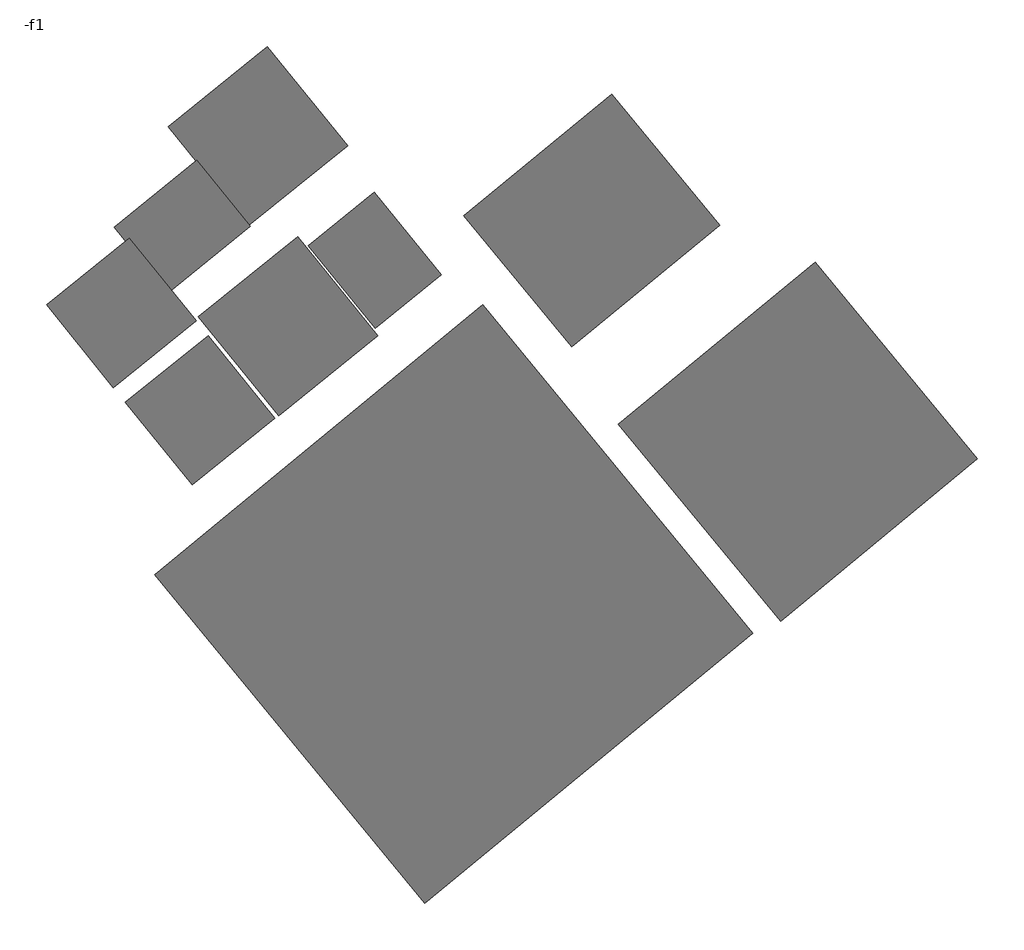
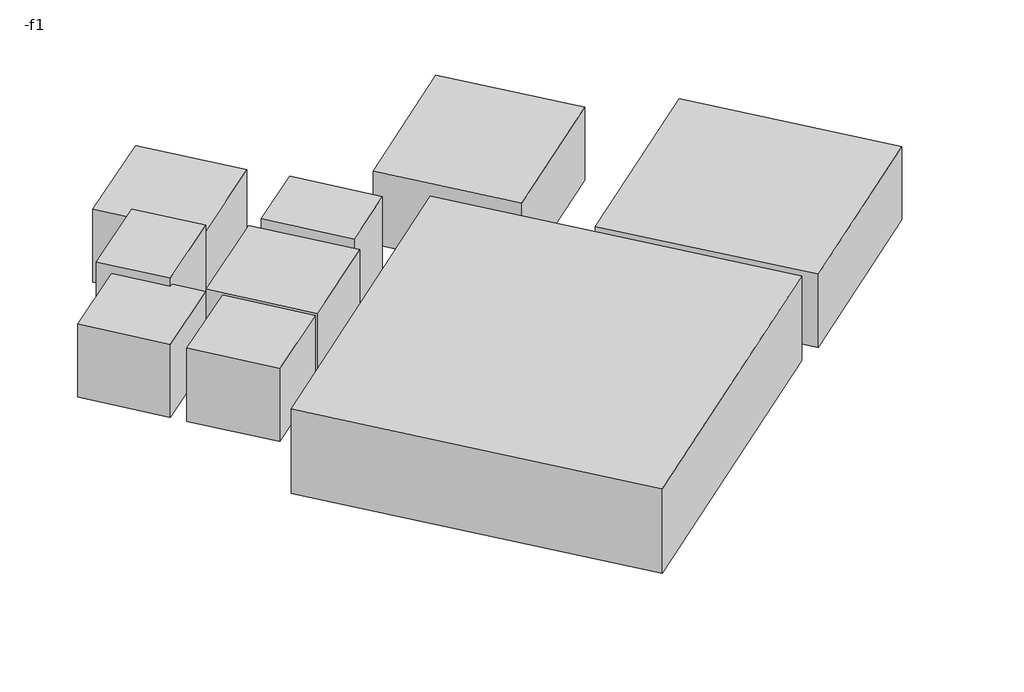
# One storey: 9 proxies.
"""IFC4 building model written with IfcOpenShell, lengths in millimetres."""

from ifc_helpers import new_model, si_unit, frame, origin, place, context, project, spatial, polyline, outline, extrude, element, save

model = new_model("IFC4")

# Units and contexts
model_context = context("Model", 3, world=origin())
ifc_project = project(units=[si_unit("LENGTHUNIT", "METRE", prefix="MILLI")], contexts=[model_context])

# Site, building, storey
site = spatial("IfcSite", under=ifc_project)
building = spatial("IfcBuilding", under=site)
storey = spatial("IfcBuildingStorey", under=building, Name="-f1", Elevation=-1400.0)

# Proxies
placement = place(None, origin())
element("IfcBuildingElementProxy", 1, Name="私有-封闭 : Supply, Equipment, and Seasonal Furniture Storage", ObjectType="私有-封闭 : Supply, Equipment, and Seasonal Furniture Storage", at=placement, inside=storey, context=model_context, shape_type="SweptSolid", body=[
    extrude(outline(polyline([(-34794.6694804, 4511.352913), (-31018.7471341, -151.5228557), (-35681.6229029, -3927.445202), (-39457.5452492, 735.4305667), (-34794.6694804, 4511.352913)])), frame((0.0, 0.0, -1400.0), z_axis=(0.0, 0.0, 1.0), x_axis=(1.0, 0.0, 0.0)), (0.0, 0.0, 1.0), 4500.0),
])
element("IfcBuildingElementProxy", 2, Name="私有-封闭 : Landscape and Grounds Maintenance Equipment Storage", ObjectType="私有-封闭 : Landscape and Grounds Maintenance Equipment Storage", at=placement, inside=storey, context=model_context, shape_type="SweptSolid", body=[
    extrude(outline(polyline([(-39005.8178352, -144.9924785), (-35859.2158799, -4030.7222858), (-39744.9456872, -7177.3242411), (-42891.5476425, -3291.5944338), (-39005.8178352, -144.9924785)])), frame((0.0, 0.0, -1400.0), z_axis=(0.0, 0.0, 1.0), x_axis=(1.0, 0.0, 0.0)), (0.0, 0.0, 1.0), 4500.0),
])
element("IfcBuildingElementProxy", 3, Name="临时私有-开敞 : IT Server, Workroom and Staff Offices", ObjectType="临时私有-开敞 : IT Server, Workroom and Staff Offices", at=placement, inside=storey, context=model_context, shape_type="SweptSolid", body=[
    extrude(outline(polyline([(-36216.5856453, 13452.3157929), (-32440.663299, 8789.4400242), (-37103.5390677, 5013.5176779), (-40879.461414, 9676.3934466), (-36216.5856453, 13452.3157929)])), frame((0.0, 0.0, -1400.0), z_axis=(0.0, 0.0, 1.0), x_axis=(1.0, 0.0, 0.0)), (0.0, 0.0, 1.0), 4500.0),
])
element("IfcBuildingElementProxy", 4, Name="临时私有-开敞 : Custodial Office", ObjectType="临时私有-开敞 : Custodial Office", at=placement, inside=storey, context=model_context, shape_type="SweptSolid", body=[
    extrude(outline(polyline([(-39531.1745049, 8096.0214901), (-37013.8929407, 4987.4376443), (-40899.622748, 1840.835689), (-43416.9043122, 4949.4195349), (-39531.1745049, 8096.0214901)])), frame((0.0, 0.0, -1400.0), z_axis=(0.0, 0.0, 1.0), x_axis=(1.0, 0.0, 0.0)), (0.0, 0.0, 1.0), 5000.0),
])
element("IfcBuildingElementProxy", 5, Name="私有-封闭 : Electrical", ObjectType="私有-封闭 : Electrical", at=placement, inside=storey, context=model_context, shape_type="SweptSolid", body=[
    extrude(outline(polyline([(-20018.4686757, 11213.5389154), (-14935.0026254, 5036.2925292), (-21884.4048099, -682.6067774), (-26967.8708601, 5494.6396088), (-20018.4686757, 11213.5389154)])), frame((0.0, 0.0, -1400.0), z_axis=(0.0, 0.0, 1.0), x_axis=(1.0, 0.0, 0.0)), (0.0, 0.0, 1.0), 4500.0),
])
element("IfcBuildingElementProxy", 6, Name="临时私有-封闭 : Kitchen", ObjectType="临时私有-封闭 : Kitchen", at=placement, inside=storey, context=model_context, shape_type="SweptSolid", body=[
    extrude(outline(polyline([(-41521.3937811, -11411.5838445), (-26078.2778156, 1297.0812812), (-13369.6126899, -14146.0346843), (-28812.7286554, -26854.69981), (-41521.3937811, -11411.5838445)])), frame((0.0, 0.0, -1400.0), z_axis=(0.0, 0.0, 1.0), x_axis=(1.0, 0.0, 0.0)), (0.0, 0.0, 1.0), 5200.0),
])
element("IfcBuildingElementProxy", 7, Name="私有-封闭 : Locker Rooms", ObjectType="私有-封闭 : Locker Rooms", at=placement, inside=storey, context=model_context, shape_type="SweptSolid", body=[
    extrude(outline(polyline([(-42718.8081424, 4440.1686941), (-39572.2061871, 554.4388868), (-43457.9359944, -2592.1630685), (-46604.5379496, 1293.5667388), (-42718.8081424, 4440.1686941)])), frame((0.0, 0.0, -1400.0), z_axis=(0.0, 0.0, 1.0), x_axis=(1.0, 0.0, 0.0)), (0.0, 0.0, 1.0), 4500.0),
])
element("IfcBuildingElementProxy", 8, Name="私有-封闭 : Mechanical", ObjectType="私有-封闭 : Mechanical", at=placement, inside=storey, context=model_context, shape_type="SweptSolid", body=[
    extrude(outline(polyline([(-10427.9993888, 3311.8372022), (-2802.8003134, -5954.032377), (-12068.6698927, -13579.2314525), (-19693.8689681, -4313.3618732), (-10427.9993888, 3311.8372022)])), frame((0.0, 0.0, -1400.0), z_axis=(0.0, 0.0, 1.0), x_axis=(1.0, 0.0, 0.0)), (0.0, 0.0, 1.0), 4500.0),
])
element("IfcBuildingElementProxy", 9, Name="私有-封闭 : Security Office/Control Room", ObjectType="私有-封闭 : Security Office/Control Room", at=placement, inside=storey, context=model_context, shape_type="SweptSolid", body=[
    extrude(outline(polyline([(-34294.9149459, 4083.3490204), (-31186.3311001, 6600.6305846), (-28039.7291448, 2714.9007773), (-31148.3129906, 197.6192131), (-34294.9149459, 4083.3490204)])), frame((0.0, 0.0, -1400.0), z_axis=(0.0, 0.0, 1.0), x_axis=(1.0, 0.0, 0.0)), (0.0, 0.0, 1.0), 5000.0),
])

save(model, "model.ifc")

# Revit data of these elements
# Project information
#   项目发布日期 = "出图日期"
#   项目状态 = "项目状态"
#   客户姓名 = "所有者"
#   项目地址 = "请在此处输入地址"
#   项目名称 = "项目名称"
#   项目编号 = "项目编号"
# Grids (mm)
#   "2": line (19783.264, -119869.538) -> (-91877.128, 61995.876)
# Type "私有-封闭 : Supply, Equipment, and Seasonal Furniture Storage"
#   Default Elevation = 1219.2 mm
#   私有_封闭_房间_面积 = 36.00 m²
#   私有_封闭_房间_进深 = 6000 mm
#   私有_封闭_房间_开间 = 6000 mm
#   私有_封闭_房间_层高 = 4500 mm
# Type "私有-封闭 : Landscape and Grounds Maintenance Equipment Storage"
#   Default Elevation = 1219.2 mm
#   私有_封闭_房间_面积 = 25.00 m²
#   私有_封闭_房间_进深 = 5000 mm
#   私有_封闭_房间_开间 = 5000 mm
#   私有_封闭_房间_层高 = 4500 mm
# Type "临时私有-开敞 : IT Server, Workroom and Staff Offices"
#   Default Elevation = 1219.2 mm
#   公共_封闭_房间_面积 = 36.00 m²
#   临时私有_开敞_房间_进深 = 6000 mm
#   临时私有_开敞_房间_开间 = 6000 mm
#   临时私有_开敞_房间_层高 = 4500 mm
# Type "临时私有-开敞 : Custodial Office"
#   Default Elevation = 1219.2 mm
#   公共_封闭_房间_面积 = 20.00 m²
#   临时私有_开敞_房间_进深 = 4000 mm
#   临时私有_开敞_房间_开间 = 5000 mm
#   临时私有_开敞_房间_层高 = 5000 mm
# Type "私有-封闭 : Electrical"
#   Default Elevation = 1219.2 mm
#   私有_封闭_房间_面积 = 72.00 m²
#   私有_封闭_房间_进深 = 8000 mm
#   私有_封闭_房间_开间 = 9000 mm
#   私有_封闭_房间_层高 = 4500 mm
# Type "临时私有-封闭 : Kitchen"
#   Default Elevation = 1219.2 mm
#   临时私有_封闭_房间_面积 = 400.00 m²
#   临时私有_封闭_房间_进深 = 20000 mm
#   临时私有_封闭_房间_开间 = 20000 mm
#   临时私有_封闭_房间_层高 = 5200 mm
# Type "私有-封闭 : Locker Rooms"
#   Default Elevation = 1219.2 mm
#   私有_封闭_房间_面积 = 25.00 m²
#   私有_封闭_房间_进深 = 5000 mm
#   私有_封闭_房间_开间 = 5000 mm
#   私有_封闭_房间_层高 = 4500 mm
# Type "私有-封闭 : Mechanical"
#   Default Elevation = 1219.2 mm
#   私有_封闭_房间_面积 = 144.00 m²
#   私有_封闭_房间_进深 = 12000 mm
#   私有_封闭_房间_开间 = 12000 mm
#   私有_封闭_房间_层高 = 4500 mm
# Type "私有-封闭 : Security Office/Control Room"
#   Default Elevation = 1219.2 mm
#   私有_封闭_房间_面积 = 20.00 m²
#   私有_封闭_房间_进深 = 4000 mm
#   私有_封闭_房间_开间 = 5000 mm
#   私有_封闭_房间_层高 = 5000 mm
# Element 1 (IfcBuildingElementProxy, "私有-封闭 : Supply, Equipment, and Seasonal Furniture Storage")
#   Phase Created = 新构造
#   Materials on its faces: "私有_封闭_房间"
# Element 2 (IfcBuildingElementProxy, "私有-封闭 : Landscape and Grounds Maintenance Equipment Storage")
#   Phase Created = 新构造
#   Materials on its faces: "私有_封闭_房间"
# Element 3 (IfcBuildingElementProxy, "临时私有-开敞 : IT Server, Workroom and Staff Offices")
#   Phase Created = 新构造
#   Materials on its faces: "临时私有_开敞_房间"
# Element 4 (IfcBuildingElementProxy, "临时私有-开敞 : Custodial Office")
#   Phase Created = 新构造
#   Materials on its faces: "临时私有_开敞_房间"
# Element 5 (IfcBuildingElementProxy, "私有-封闭 : Electrical")
#   Phase Created = 新构造
#   Materials on its faces: "私有_封闭_房间"
# Element 6 (IfcBuildingElementProxy, "临时私有-封闭 : Kitchen")
#   Phase Created = 新构造
#   Materials on its faces: "临时私有_封闭_房间"
# Element 7 (IfcBuildingElementProxy, "私有-封闭 : Locker Rooms")
#   Phase Created = 新构造
#   Materials on its faces: "私有_封闭_房间"
# Element 8 (IfcBuildingElementProxy, "私有-封闭 : Mechanical")
#   Phase Created = 新构造
#   Materials on its faces: "私有_封闭_房间"
# Element 9 (IfcBuildingElementProxy, "私有-封闭 : Security Office/Control Room")
#   Phase Created = 新构造
#   Materials on its faces: "私有_封闭_房间"
# Materials
#   "私有_封闭_房间": class "其他", colour RGB 81 40 0, transparency 0
#   "临时私有_开敞_房间": class "玻璃", colour RGB 206 67 0, transparency 0
#   "临时私有_封闭_房间": class "其他", colour RGB 77 38 0, transparency 0
